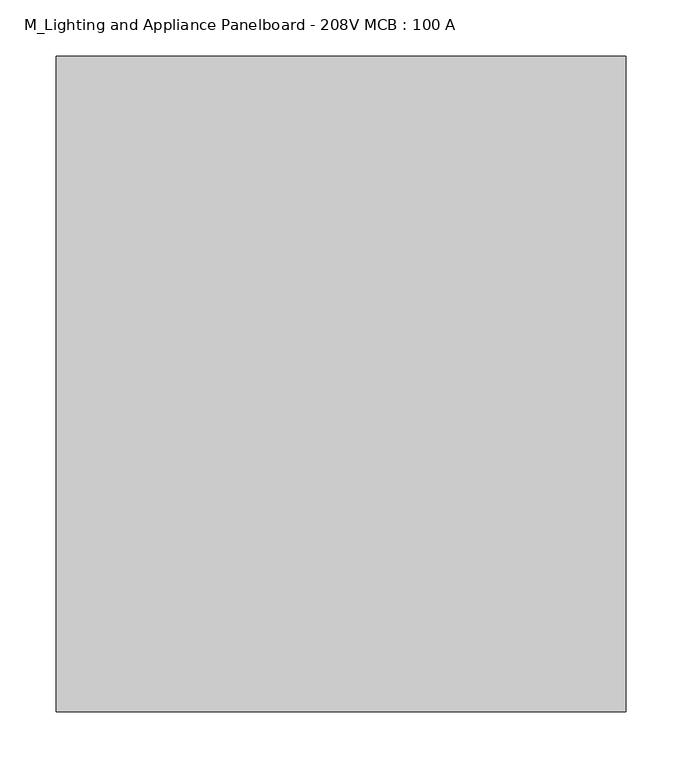
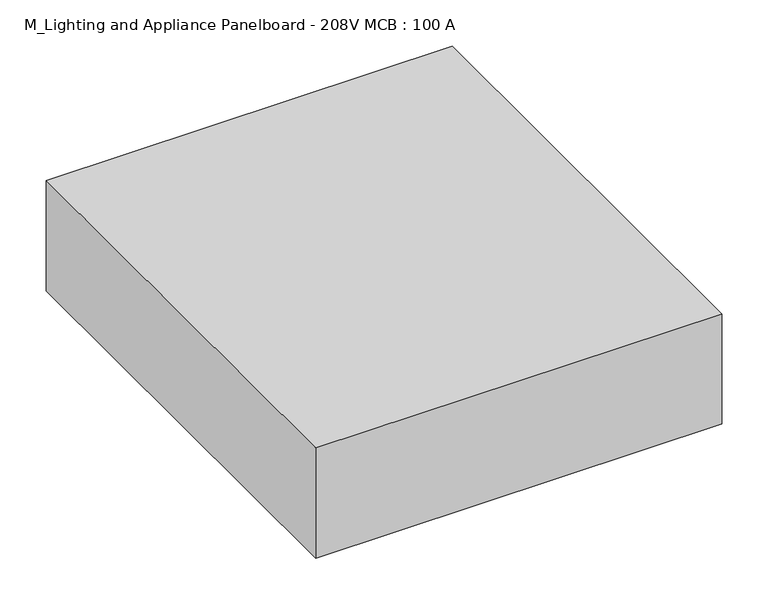
"""IFC4 building model written with IfcOpenShell, lengths in millimetres: proxy geometry, M_Lighting and Appliance Panelboard - 208V MCB : 100 A."""

from ifc_helpers import new_model, si_unit, frame, origin, place, context, project, spatial, polyline, outline, extrude, source, transform, mapped, element, save


def m_lighting_and_appliance_panelboard_208v_mcb_100_a_1c5cc82c(model_context):
    return source(origin(), model_context, "Body", "SweptSolid", [
        extrude(outline(polyline([(349.2594706, 55.9943297), (349.2594706, -528.2056703), (-158.7405294, -528.2056703), (-158.7405294, 55.9943297), (349.2594706, 55.9943297)])), frame((0.0, 0.0, -146.1), z_axis=(0.0, 0.0, 1.0), x_axis=(1.0, 0.0, 0.0)), (0.0, 0.0, 1.0), 146.1),
    ])


if __name__ == "__main__":
    model = new_model("IFC4")
    model_context = context("Model", 3, world=origin())
    ifc_project = project(units=[si_unit("LENGTHUNIT", "METRE", prefix="MILLI")], contexts=[model_context])
    site = spatial("IfcSite", under=ifc_project)
    building = spatial("IfcBuilding", under=site)
    placement = place(None, origin())
    m_lighting_and_appliance_panelboard_208v_mcb_100_a_shape = m_lighting_and_appliance_panelboard_208v_mcb_100_a_1c5cc82c(model_context)
    element("IfcBuildingElementProxy", 1, Name="M_Lighting and Appliance Panelboard - 208V MCB : 100 A", ObjectType="M_Lighting and Appliance Panelboard - 208V MCB : 100 A", at=placement, inside=building, context=model_context, shape_type="MappedRepresentation", body=[
        mapped(m_lighting_and_appliance_panelboard_208v_mcb_100_a_shape, transform((0.0, 0.0, 0.0), x_axis=(1.0, 0.0, 0.0), y_axis=(0.0, 1.0, 0.0), z_axis=(0.0, 0.0, 1.0))),
    ])
    save(model, "model.ifc")

# Revit data of these elements
# Type "M_Lighting and Appliance Panelboard - 208V MCB : 100 A"
#   built-in parameter 1140081 [instance default] = "Recessed"
#   built-in parameter 1140083 [instance default] = "Type 1"
#   Width = 508 mm
#   built-in parameter 1140082 [instance default] = 100 (stored number, unit not read)
#   built-in parameter 1140140 = 100 (stored number, unit not read)
#   Height [instance default] = 584.2 mm
#   Depth = 146.1 mm
#   Default Elevation = 1200 mm
#   42 Circuit Height = 1270 mm
#   30 Circuit Height = 736.6 mm
#   24 Circuit Height = 660.4 mm
#   12 Circuit Height = 584.2 mm
#   built-in parameter 1140079 [instance default] = 12
#   Load Classification = Other
